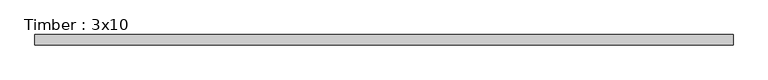
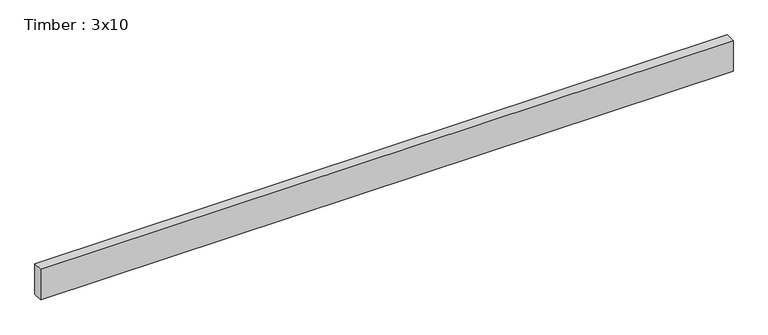
"""IFC4 building model written with IfcOpenShell, lengths in millimetres: beam geometry, Timber : 3x10."""

from ifc_helpers import new_model, si_unit, frame, origin, place, context, project, spatial, polyline, outline, extrude, source, transform, mapped, element, save


def timber_3x10_fcfe8c29(model_context):
    return source(origin(), model_context, "Body", "SweptSolid", [
        extrude(outline(polyline([(2603.5, 38.1), (2603.5, -38.1), (-2603.5, -38.1), (-2603.5, 38.1), (2603.5, 38.1)])), frame((0.0, 0.0, -120.65), z_axis=(0.0, 0.0, 1.0), x_axis=(1.0, 0.0, 0.0)), (0.0, 0.0, 1.0), 241.3),
    ])


if __name__ == "__main__":
    model = new_model("IFC4")
    model_context = context("Model", 3, world=origin())
    ifc_project = project(units=[si_unit("LENGTHUNIT", "METRE", prefix="MILLI")], contexts=[model_context])
    site = spatial("IfcSite", under=ifc_project)
    building = spatial("IfcBuilding", under=site)
    placement = place(None, origin())
    timber_3x10_shape = timber_3x10_fcfe8c29(model_context)
    element("IfcBeam", 1, ObjectType="Timber : 3x10", at=placement, inside=building, context=model_context, shape_type="MappedRepresentation", body=[
        mapped(timber_3x10_shape, transform((0.0, 0.0, 0.0), x_axis=(1.0, 0.0, 0.0), y_axis=(0.0, 1.0, 0.0), z_axis=(0.0, 0.0, 1.0))),
    ])
    save(model, "model.ifc")

# Revit data of these elements
# Type "Timber : 3x10"
#   Assembly Code = "B10"
#   A = 0.362847 SF
#   Length [instance default] = 5' - 0"
#   b = 0' - 3"
#   d = 0' - 9 1/2"
#   Structural Material [instance default] = Softwood, Lumber
# Element 1 (IfcBeam, "Timber : 3x10")
#   Materials on its faces: "Softwood, Lumber"
# Materials
#   "Softwood, Lumber": class "Wood", colour RGB 144 113 62, transparency 0, Description = "Pinus Echinata", Cost = 0
